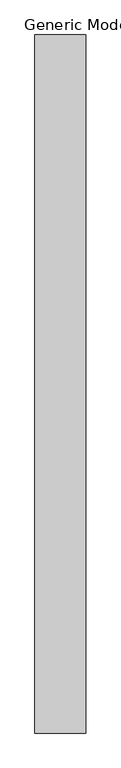
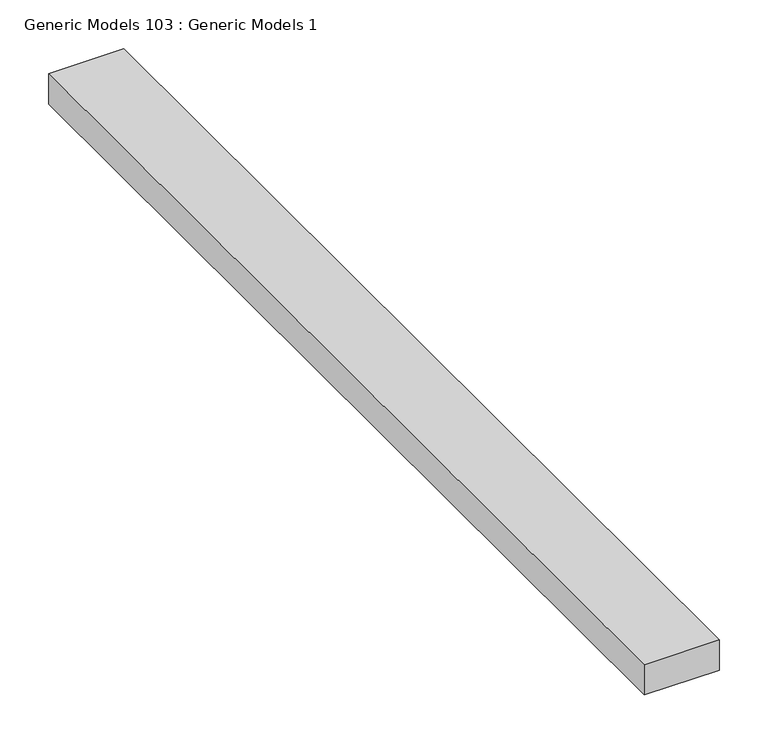
"""IFC4 building model written with IfcOpenShell, lengths in millimetres: proxy geometry, Generic Models 103 : Generic Models 1."""

from ifc_helpers import new_model, si_unit, frame, origin, place, context, project, spatial, polyline, outline, extrude, source, transform, mapped, element, save


def generic_models_103_generic_models_1_250a6a11(model_context):
    return source(origin(), model_context, "Body", "SweptSolid", [
        extrude(outline(polyline([(49784.0, 0.0), (49695.1, 0.0), (49695.1, 1219.2), (49784.0, 1219.2), (49784.0, 0.0)])), frame((0.0, 0.0, 5264.15), z_axis=(0.0, 0.0, 1.0), x_axis=(1.0, 0.0, 0.0)), (0.0, 0.0, 1.0), 38.1),
    ])


if __name__ == "__main__":
    model = new_model("IFC4")
    model_context = context("Model", 3, world=origin())
    ifc_project = project(units=[si_unit("LENGTHUNIT", "METRE", prefix="MILLI")], contexts=[model_context])
    site = spatial("IfcSite", under=ifc_project)
    building = spatial("IfcBuilding", under=site)
    placement = place(None, origin())
    generic_models_103_generic_models_1_shape = generic_models_103_generic_models_1_250a6a11(model_context)
    element("IfcBuildingElementProxy", 1, Name="Generic Models 103 : Generic Models 1", ObjectType="Generic Models 103 : Generic Models 1", at=placement, inside=building, context=model_context, shape_type="MappedRepresentation", body=[
        mapped(generic_models_103_generic_models_1_shape, transform((0.0, 0.0, 0.0), x_axis=(1.0, 0.0, 0.0), y_axis=(0.0, 1.0, 0.0), z_axis=(0.0, 0.0, 1.0))),
    ])
    save(model, "model.ifc")

# Revit data of these elements
# Element 1 (IfcBuildingElementProxy, "Generic Models 103 : Generic Models 1")
#   Materials on its faces: "2X WOOD HEADER ATTACHED TO STEEL PURLIN"
# Materials
#   "2X WOOD HEADER ATTACHED TO STEEL PURLIN": class "Wood", colour RGB 234 198 147, transparency 0, Description = "Pinus Echinata", Cost = 0
